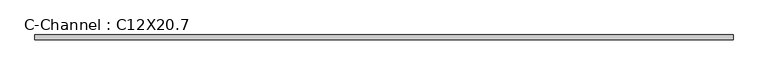
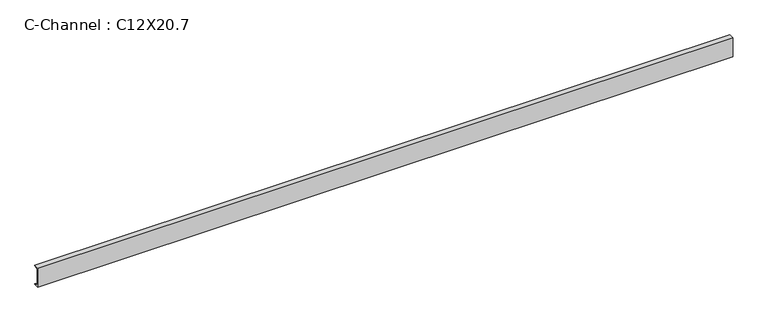
"""IFC4 building model written with IfcOpenShell, lengths in millimetres: beam geometry, C-Channel : C12X20.7."""

from ifc_helpers import new_model, si_unit, point, frame, frame_2d, origin, place, context, project, spatial, polyline, circle_curve, trimmed, segment, composite_curve, outline, extrude, source, transform, mapped, element, save


def c_channel_c12x20_7_7dff1778(model_context):
    return source(origin(), model_context, "Body", "SweptSolid", [
        extrude(outline(composite_curve([segment(polyline([(-17.7292, 152.4), (56.9468, 152.4)]), True, "CONTINUOUS"), segment(trimmed(circle_curve(frame_2d((44.2214, 152.4)), 12.7254), [point((56.9468, 152.4))], [point((44.2214, 139.6746))], False, "CARTESIAN"), True, "CONTINUOUS"), segment(polyline([(44.2214, 139.6746), (-10.5664, 130.997065), (-10.5664, -130.997065), (44.2214, -139.6746)]), True, "CONTINUOUS"), segment(trimmed(circle_curve(frame_2d((44.2214, -152.4)), 12.7254), [point((44.2214, -139.6746))], [point((56.9468, -152.4))], False, "CARTESIAN"), True, "CONTINUOUS"), segment(polyline([(56.9468, -152.4), (-17.7292, -152.4), (-17.7292, 152.4)]), True, "CONTINUOUS")], self_intersect=False)), frame((-5302.4661418, 0.0, 0.0), z_axis=(1.0, 0.0, 0.0), x_axis=(0.0, 1.0, 0.0)), (0.0, 0.0, 1.0), 10505.8999404),
    ])


if __name__ == "__main__":
    model = new_model("IFC4")
    model_context = context("Model", 3, world=origin())
    ifc_project = project(units=[si_unit("LENGTHUNIT", "METRE", prefix="MILLI")], contexts=[model_context])
    site = spatial("IfcSite", under=ifc_project)
    building = spatial("IfcBuilding", under=site)
    placement = place(None, origin())
    c_channel_c12x20_7_shape = c_channel_c12x20_7_7dff1778(model_context)
    element("IfcBeam", 1, ObjectType="C-Channel : C12X20.7", at=placement, inside=building, context=model_context, shape_type="MappedRepresentation", body=[
        mapped(c_channel_c12x20_7_shape, transform((0.0, 0.0, 0.0), x_axis=(1.0, 0.0, 0.0), y_axis=(0.0, 1.0, 0.0), z_axis=(0.0, 0.0, 1.0))),
    ])
    save(model, "model.ifc")

# Revit data of these elements
# Type "C-Channel : C12X20.7"
#   Assembly Code = "B10"
#   W = 20.7
#   Start Extension Calculation [instance default] = 10' - 0"
#   Start Extension [instance default] = -0' - 0 1/2"
#   End Extension Calculation [instance default] = 10' - 0"
#   End Extension [instance default] = -0' - 0 1/2"
#   Length [instance default] = 5' - 0"
#   bf = 0' - 2.94"
#   d = 1' - 0"
#   tf = 0' - 0.501"
#   tw = 0' - 0.282"
#   x = 0' - 0.698"
#   A = 0.0422222 SF
#   Structural Material [instance default] = Metal - Steel - ASTM A36
# Element 1 (IfcBeam, "C-Channel : C12X20.7")
#   Materials on its faces: "Metal - Steel - ASTM A36"
# Materials
#   "Metal - Steel - ASTM A36": class "Metal", colour RGB 199 199 199, transparency 0
